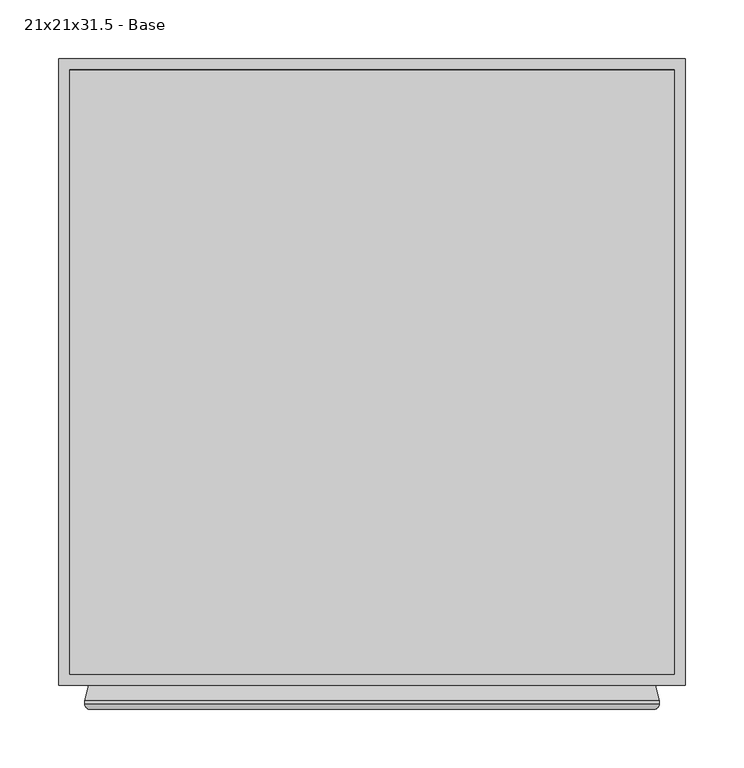
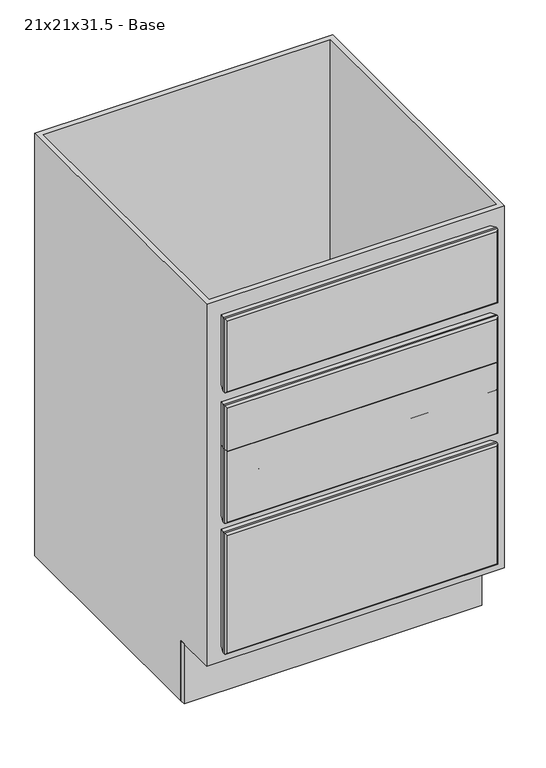
"""IFC4 building model written with IfcOpenShell, lengths in millimetres: furniture geometry, Cabinet-Base-Merillat-Four_Drawer-Marlin : 21x21x31.5 - Base."""

from ifc_helpers import new_model, si_unit, frame, origin, origin_with_axes, place, context, project, spatial, polyline, ellipse_curve, outline, extrude, faceted_brep, source, transform, mapped, element, save
from ifc_brep_helpers import plane_surface, cylinder_surface, advanced_brep


def furniture_21x21x31_5_base_fe1b8182(model_context):
    return source(origin(), model_context, "Body", "SolidModel", [
        advanced_brep(
        [(-222.6408026, -629.92, 365.2035075), (-222.6408026, -629.92, 142.7964925), (260.1162124, -629.92, 142.7964925), (260.1162124, -629.92, 365.2035075), (-222.2320951, -609.6, 143.2052), (-222.2320951, -609.6, 364.7948), (259.7075049, -609.6, 364.7948), (259.7075049, -609.6, 143.2052), (-225.7372951, -625.4496, 368.3), (-225.7372951, -622.681, 368.3), (-225.7372951, -622.681, 139.7), (-225.7372951, -625.4496, 139.7), (263.2127049, -622.681, 139.7), (263.2127049, -625.4496, 139.7), (263.2127049, -622.681, 368.3), (263.2127049, -625.4496, 368.3)],
        [
            (0, 1),
            (1, 2),
            (2, 3),
            (3, 0),
            (4, 5),
            (5, 6),
            (6, 7),
            (7, 4),
            (8, 9),
            (9, 10),
            (10, 11),
            (11, 8),
            (10, 12),
            (12, 13),
            (13, 11),
            (12, 14),
            (14, 15),
            (15, 13),
            (8, 15),
            (14, 9),
            (11, 1, ellipse_curve(frame((-220.9620951, -625.4496, 144.4752), z_axis=(-0.7071067811865475, 0.0, 0.7071067811865475), x_axis=(-0.7071067811865474, 0.0, -0.7071067811865476)), 6.7531526, 4.7752)),
            (0, 8, ellipse_curve(frame((-220.9620951, -625.4496, 363.5248), z_axis=(-0.7071067811865475, 0.0, -0.7071067811865475), x_axis=(0.7071067811865474, 0.0, -0.7071067811865476)), 6.7531526, 4.7752)),
            (4, 10),
            (9, 5),
            (13, 2, ellipse_curve(frame((258.4375049, -625.4496, 144.4752), z_axis=(-0.7071067811865475, 0.0, -0.7071067811865475), x_axis=(0.7071067811865476, 0.0, -0.7071067811865474)), 6.7531526, 4.7752)),
            (7, 12),
            (15, 3, ellipse_curve(frame((258.4375049, -625.4496, 363.5248), z_axis=(0.7071067811865475, 0.0, -0.7071067811865475), x_axis=(0.7071067811865474, 0.0, 0.7071067811865476)), 6.7531526, 4.7752)),
            (6, 14),
        ],
        [
            plane_surface(frame((-225.7372951, -629.92, 368.3), z_axis=(0.0, -1.0, 0.0), x_axis=(0.0, 0.0, -1.0))),
            plane_surface(frame((-225.7372951, -609.6, 368.3), z_axis=(0.0, 1.0, 0.0), x_axis=(0.0, 0.0, 1.0))),
            plane_surface(frame((-225.7372951, -629.92, 368.3), z_axis=(-1.0, 0.0, 0.0), x_axis=(0.0, 1.0, 0.0))),
            plane_surface(frame((-225.7372951, -629.92, 139.7), z_axis=(0.0, 0.0, -1.0), x_axis=(0.0, 1.0, 0.0))),
            plane_surface(frame((263.2127049, -629.92, 139.7), z_axis=(1.0, 0.0, 0.0), x_axis=(0.0, 1.0, 0.0))),
            plane_surface(frame((263.2127049, -629.92, 368.3), z_axis=(0.0, 0.0, 1.0), x_axis=(0.0, 1.0, 0.0))),
            cylinder_surface(frame((-220.9620951, -625.4496, 368.3), z_axis=(0.0, 0.0, -1.0), x_axis=(0.0, 1.0, 0.0)), 4.7752),
            plane_surface(frame((-225.7372951, -622.681, 368.3), z_axis=(-0.9659229350723619, 0.25882983502910506, 0.0), x_axis=(0.0, 0.0, -1.0))),
            cylinder_surface(frame((-225.7372951, -625.4496, 144.4752), z_axis=(1.0, 0.0, 0.0), x_axis=(0.0, 1.0, 0.0)), 4.7752),
            plane_surface(frame((-225.7372951, -622.681, 139.7), z_axis=(0.0, 0.25882983502910506, -0.9659229350723619), x_axis=(1.0, 0.0, 0.0))),
            cylinder_surface(frame((258.4375049, -625.4496, 139.7), z_axis=(0.0, 0.0, 1.0), x_axis=(0.0, 1.0, 0.0)), 4.7752),
            plane_surface(frame((263.2127049, -622.681, 139.7), z_axis=(0.9659229350723619, 0.25882983502910506, 0.0), x_axis=(0.0, 0.0, 1.0))),
            cylinder_surface(frame((263.2127049, -625.4496, 363.5248), z_axis=(-1.0, 0.0, 0.0), x_axis=(0.0, 1.0, 0.0)), 4.7752),
            plane_surface(frame((263.2127049, -622.681, 368.3), z_axis=(0.0, 0.25882983502910506, 0.9659229350723619), x_axis=(-1.0, 0.0, 0.0))),
        ],
        [
            (0, [[1, 2, 3, 4]]),
            (1, [[5, 6, 7, 8]]),
            (2, [[9, 10, 11, 12]]),
            (3, [[-11, 13, 14, 15]]),
            (4, [[-14, 16, 17, 18]]),
            (5, [[-9, 19, -17, 20]]),
            (6, [[21, -1, 22, -12]]),
            (7, [[23, -10, 24, -5]]),
            (8, [[-21, -15, 25, -2]]),
            (9, [[-23, -8, 26, -13]]),
            (10, [[-25, -18, 27, -3]]),
            (11, [[-26, -7, 28, -16]]),
            (12, [[-22, -4, -27, -19]]),
            (13, [[-24, -20, -28, -6]]),
        ],
    ),
        advanced_brep(
        [(-222.6408026, -629.92, 523.9535075), (-222.6408026, -629.92, 390.4464925), (260.1162124, -629.92, 390.4464925), (260.1162124, -629.92, 523.9535075), (-222.2320951, -609.6, 390.8552), (-222.2320951, -609.6, 523.5448), (259.7075049, -609.6, 523.5448), (259.7075049, -609.6, 390.8552), (-225.7372951, -625.4496, 527.05), (-225.7372951, -622.681, 527.05), (-225.7372951, -622.681, 387.35), (-225.7372951, -625.4496, 387.35), (263.2127049, -622.681, 387.35), (263.2127049, -625.4496, 387.35), (263.2127049, -622.681, 527.05), (263.2127049, -625.4496, 527.05)],
        [
            (0, 1),
            (1, 2),
            (2, 3),
            (3, 0),
            (4, 5),
            (5, 6),
            (6, 7),
            (7, 4),
            (8, 9),
            (9, 10),
            (10, 11),
            (11, 8),
            (10, 12),
            (12, 13),
            (13, 11),
            (12, 14),
            (14, 15),
            (15, 13),
            (8, 15),
            (14, 9),
            (11, 1, ellipse_curve(frame((-220.9620951, -625.4496, 392.1252), z_axis=(-0.7071067811865475, 0.0, 0.7071067811865475), x_axis=(-0.7071067811865474, 0.0, -0.7071067811865476)), 6.7531526, 4.7752)),
            (0, 8, ellipse_curve(frame((-220.9620951, -625.4496, 522.2748), z_axis=(-0.7071067811865475, 0.0, -0.7071067811865475), x_axis=(0.7071067811865474, 0.0, -0.7071067811865476)), 6.7531526, 4.7752)),
            (4, 10),
            (9, 5),
            (13, 2, ellipse_curve(frame((258.4375049, -625.4496, 392.1252), z_axis=(-0.7071067811865475, 0.0, -0.7071067811865475), x_axis=(0.7071067811865476, 0.0, -0.7071067811865474)), 6.7531526, 4.7752)),
            (7, 12),
            (15, 3, ellipse_curve(frame((258.4375049, -625.4496, 522.2748), z_axis=(0.7071067811865475, 0.0, -0.7071067811865475), x_axis=(0.7071067811865474, 0.0, 0.7071067811865476)), 6.7531526, 4.7752)),
            (6, 14),
        ],
        [
            plane_surface(frame((-225.7372951, -629.92, 527.05), z_axis=(0.0, -1.0, 0.0), x_axis=(0.0, 0.0, -1.0))),
            plane_surface(frame((-225.7372951, -609.6, 527.05), z_axis=(0.0, 1.0, 0.0), x_axis=(0.0, 0.0, 1.0))),
            plane_surface(frame((-225.7372951, -629.92, 527.05), z_axis=(-1.0, 0.0, 0.0), x_axis=(0.0, 1.0, 0.0))),
            plane_surface(frame((-225.7372951, -629.92, 387.35), z_axis=(0.0, 0.0, -1.0), x_axis=(0.0, 1.0, 0.0))),
            plane_surface(frame((263.2127049, -629.92, 387.35), z_axis=(1.0, 0.0, 0.0), x_axis=(0.0, 1.0, 0.0))),
            plane_surface(frame((263.2127049, -629.92, 527.05), z_axis=(0.0, 0.0, 1.0), x_axis=(0.0, 1.0, 0.0))),
            cylinder_surface(frame((-220.9620951, -625.4496, 527.05), z_axis=(0.0, 0.0, -1.0), x_axis=(0.0, 1.0, 0.0)), 4.7752),
            plane_surface(frame((-225.7372951, -622.681, 527.05), z_axis=(-0.9659229350723619, 0.25882983502910506, 0.0), x_axis=(0.0, 0.0, -1.0))),
            cylinder_surface(frame((-225.7372951, -625.4496, 392.1252), z_axis=(1.0, 0.0, 0.0), x_axis=(0.0, 1.0, 0.0)), 4.7752),
            plane_surface(frame((-225.7372951, -622.681, 387.35), z_axis=(0.0, 0.25882983502910506, -0.9659229350723619), x_axis=(1.0, 0.0, 0.0))),
            cylinder_surface(frame((258.4375049, -625.4496, 387.35), z_axis=(0.0, 0.0, 1.0), x_axis=(0.0, 1.0, 0.0)), 4.7752),
            plane_surface(frame((263.2127049, -622.681, 387.35), z_axis=(0.9659229350723619, 0.25882983502910506, 0.0), x_axis=(0.0, 0.0, 1.0))),
            cylinder_surface(frame((263.2127049, -625.4496, 522.2748), z_axis=(-1.0, 0.0, 0.0), x_axis=(0.0, 1.0, 0.0)), 4.7752),
            plane_surface(frame((263.2127049, -622.681, 527.05), z_axis=(0.0, 0.25882983502910506, 0.9659229350723619), x_axis=(-1.0, 0.0, 0.0))),
        ],
        [
            (0, [[1, 2, 3, 4]]),
            (1, [[5, 6, 7, 8]]),
            (2, [[9, 10, 11, 12]]),
            (3, [[-11, 13, 14, 15]]),
            (4, [[-14, 16, 17, 18]]),
            (5, [[-9, 19, -17, 20]]),
            (6, [[21, -1, 22, -12]]),
            (7, [[23, -10, 24, -5]]),
            (8, [[-21, -15, 25, -2]]),
            (9, [[-23, -8, 26, -13]]),
            (10, [[-25, -18, 27, -3]]),
            (11, [[-26, -7, 28, -16]]),
            (12, [[-22, -4, -27, -19]]),
            (13, [[-24, -20, -28, -6]]),
        ],
    ),
        advanced_brep(
        [(-222.6408026, -629.92, 606.5035075), (-222.6408026, -629.92, 472.9964925), (260.1162124, -629.92, 472.9964925), (260.1162124, -629.92, 606.5035075), (-222.2320951, -609.6, 473.4052), (-222.2320951, -609.6, 606.0948), (259.7075049, -609.6, 606.0948), (259.7075049, -609.6, 473.4052), (-225.7372951, -625.4496, 609.6), (-225.7372951, -622.681, 609.6), (-225.7372951, -622.681, 469.9), (-225.7372951, -625.4496, 469.9), (263.2127049, -622.681, 469.9), (263.2127049, -625.4496, 469.9), (263.2127049, -622.681, 609.6), (263.2127049, -625.4496, 609.6)],
        [
            (0, 1),
            (1, 2),
            (2, 3),
            (3, 0),
            (4, 5),
            (5, 6),
            (6, 7),
            (7, 4),
            (8, 9),
            (9, 10),
            (10, 11),
            (11, 8),
            (10, 12),
            (12, 13),
            (13, 11),
            (12, 14),
            (14, 15),
            (15, 13),
            (8, 15),
            (14, 9),
            (11, 1, ellipse_curve(frame((-220.9620951, -625.4496, 474.6752), z_axis=(-0.7071067811865475, 0.0, 0.7071067811865475), x_axis=(-0.7071067811865474, 0.0, -0.7071067811865476)), 6.7531526, 4.7752)),
            (0, 8, ellipse_curve(frame((-220.9620951, -625.4496, 604.8248), z_axis=(-0.7071067811865475, 0.0, -0.7071067811865475), x_axis=(0.7071067811865474, 0.0, -0.7071067811865476)), 6.7531526, 4.7752)),
            (4, 10),
            (9, 5),
            (13, 2, ellipse_curve(frame((258.4375049, -625.4496, 474.6752), z_axis=(-0.7071067811865475, 0.0, -0.7071067811865475), x_axis=(0.7071067811865476, 0.0, -0.7071067811865474)), 6.7531526, 4.7752)),
            (7, 12),
            (15, 3, ellipse_curve(frame((258.4375049, -625.4496, 604.8248), z_axis=(0.7071067811865475, 0.0, -0.7071067811865475), x_axis=(0.7071067811865474, 0.0, 0.7071067811865476)), 6.7531526, 4.7752)),
            (6, 14),
        ],
        [
            plane_surface(frame((-225.7372951, -629.92, 609.6), z_axis=(0.0, -1.0, 0.0), x_axis=(0.0, 0.0, -1.0))),
            plane_surface(frame((-225.7372951, -609.6, 609.6), z_axis=(0.0, 1.0, 0.0), x_axis=(0.0, 0.0, 1.0))),
            plane_surface(frame((-225.7372951, -629.92, 609.6), z_axis=(-1.0, 0.0, 0.0), x_axis=(0.0, 1.0, 0.0))),
            plane_surface(frame((-225.7372951, -629.92, 469.9), z_axis=(0.0, 0.0, -1.0), x_axis=(0.0, 1.0, 0.0))),
            plane_surface(frame((263.2127049, -629.92, 469.9), z_axis=(1.0, 0.0, 0.0), x_axis=(0.0, 1.0, 0.0))),
            plane_surface(frame((263.2127049, -629.92, 609.6), z_axis=(0.0, 0.0, 1.0), x_axis=(0.0, 1.0, 0.0))),
            cylinder_surface(frame((-220.9620951, -625.4496, 609.6), z_axis=(0.0, 0.0, -1.0), x_axis=(0.0, 1.0, 0.0)), 4.7752),
            plane_surface(frame((-225.7372951, -622.681, 609.6), z_axis=(-0.9659229350723619, 0.25882983502910506, 0.0), x_axis=(0.0, 0.0, -1.0))),
            cylinder_surface(frame((-225.7372951, -625.4496, 474.6752), z_axis=(1.0, 0.0, 0.0), x_axis=(0.0, 1.0, 0.0)), 4.7752),
            plane_surface(frame((-225.7372951, -622.681, 469.9), z_axis=(0.0, 0.25882983502910506, -0.9659229350723619), x_axis=(1.0, 0.0, 0.0))),
            cylinder_surface(frame((258.4375049, -625.4496, 469.9), z_axis=(0.0, 0.0, 1.0), x_axis=(0.0, 1.0, 0.0)), 4.7752),
            plane_surface(frame((263.2127049, -622.681, 469.9), z_axis=(0.9659229350723619, 0.25882983502910506, 0.0), x_axis=(0.0, 0.0, 1.0))),
            cylinder_surface(frame((263.2127049, -625.4496, 604.8248), z_axis=(-1.0, 0.0, 0.0), x_axis=(0.0, 1.0, 0.0)), 4.7752),
            plane_surface(frame((263.2127049, -622.681, 609.6), z_axis=(0.0, 0.25882983502910506, 0.9659229350723619), x_axis=(-1.0, 0.0, 0.0))),
        ],
        [
            (0, [[1, 2, 3, 4]]),
            (1, [[5, 6, 7, 8]]),
            (2, [[9, 10, 11, 12]]),
            (3, [[-11, 13, 14, 15]]),
            (4, [[-14, 16, 17, 18]]),
            (5, [[-9, 19, -17, 20]]),
            (6, [[21, -1, 22, -12]]),
            (7, [[23, -10, 24, -5]]),
            (8, [[-21, -15, 25, -2]]),
            (9, [[-23, -8, 26, -13]]),
            (10, [[-25, -18, 27, -3]]),
            (11, [[-26, -7, 28, -16]]),
            (12, [[-22, -4, -27, -19]]),
            (13, [[-24, -20, -28, -6]]),
        ],
    ),
        advanced_brep(
        [(-222.6408026, -629.92, 771.6035075), (-222.6408026, -629.92, 638.0964925), (260.1162124, -629.92, 638.0964925), (260.1162124, -629.92, 771.6035075), (-222.2320951, -609.6, 638.5052), (-222.2320951, -609.6, 771.1948), (259.7075049, -609.6, 771.1948), (259.7075049, -609.6, 638.5052), (-225.7372951, -625.4496, 774.7), (-225.7372951, -622.681, 774.7), (-225.7372951, -622.681, 635.0), (-225.7372951, -625.4496, 635.0), (263.2127049, -622.681, 635.0), (263.2127049, -625.4496, 635.0), (263.2127049, -622.681, 774.7), (263.2127049, -625.4496, 774.7)],
        [
            (0, 1),
            (1, 2),
            (2, 3),
            (3, 0),
            (4, 5),
            (5, 6),
            (6, 7),
            (7, 4),
            (8, 9),
            (9, 10),
            (10, 11),
            (11, 8),
            (10, 12),
            (12, 13),
            (13, 11),
            (12, 14),
            (14, 15),
            (15, 13),
            (8, 15),
            (14, 9),
            (11, 1, ellipse_curve(frame((-220.9620951, -625.4496, 639.7752), z_axis=(-0.7071067811865475, 0.0, 0.7071067811865475), x_axis=(-0.7071067811865474, 0.0, -0.7071067811865476)), 6.7531526, 4.7752)),
            (0, 8, ellipse_curve(frame((-220.9620951, -625.4496, 769.9248), z_axis=(-0.7071067811865475, 0.0, -0.7071067811865475), x_axis=(0.7071067811865474, 0.0, -0.7071067811865476)), 6.7531526, 4.7752)),
            (4, 10),
            (9, 5),
            (13, 2, ellipse_curve(frame((258.4375049, -625.4496, 639.7752), z_axis=(-0.7071067811865475, 0.0, -0.7071067811865475), x_axis=(0.7071067811865476, 0.0, -0.7071067811865474)), 6.7531526, 4.7752)),
            (7, 12),
            (15, 3, ellipse_curve(frame((258.4375049, -625.4496, 769.9248), z_axis=(0.7071067811865475, 0.0, -0.7071067811865475), x_axis=(0.7071067811865474, 0.0, 0.7071067811865476)), 6.7531526, 4.7752)),
            (6, 14),
        ],
        [
            plane_surface(frame((-225.7372951, -629.92, 774.7), z_axis=(0.0, -1.0, 0.0), x_axis=(0.0, 0.0, -1.0))),
            plane_surface(frame((-225.7372951, -609.6, 774.7), z_axis=(0.0, 1.0, 0.0), x_axis=(0.0, 0.0, 1.0))),
            plane_surface(frame((-225.7372951, -629.92, 774.7), z_axis=(-1.0, 0.0, 0.0), x_axis=(0.0, 1.0, 0.0))),
            plane_surface(frame((-225.7372951, -629.92, 635.0), z_axis=(0.0, 0.0, -1.0), x_axis=(0.0, 1.0, 0.0))),
            plane_surface(frame((263.2127049, -629.92, 635.0), z_axis=(1.0, 0.0, 0.0), x_axis=(0.0, 1.0, 0.0))),
            plane_surface(frame((263.2127049, -629.92, 774.7), z_axis=(0.0, 0.0, 1.0), x_axis=(0.0, 1.0, 0.0))),
            cylinder_surface(frame((-220.9620951, -625.4496, 774.7), z_axis=(0.0, 0.0, -1.0), x_axis=(0.0, 1.0, 0.0)), 4.7752),
            plane_surface(frame((-225.7372951, -622.681, 774.7), z_axis=(-0.9659229350723619, 0.25882983502910506, 0.0), x_axis=(0.0, 0.0, -1.0))),
            cylinder_surface(frame((-225.7372951, -625.4496, 639.7752), z_axis=(1.0, 0.0, 0.0), x_axis=(0.0, 1.0, 0.0)), 4.7752),
            plane_surface(frame((-225.7372951, -622.681, 635.0), z_axis=(0.0, 0.25882983502910506, -0.9659229350723619), x_axis=(1.0, 0.0, 0.0))),
            cylinder_surface(frame((258.4375049, -625.4496, 635.0), z_axis=(0.0, 0.0, 1.0), x_axis=(0.0, 1.0, 0.0)), 4.7752),
            plane_surface(frame((263.2127049, -622.681, 635.0), z_axis=(0.9659229350723619, 0.25882983502910506, 0.0), x_axis=(0.0, 0.0, 1.0))),
            cylinder_surface(frame((263.2127049, -625.4496, 769.9248), z_axis=(-1.0, 0.0, 0.0), x_axis=(0.0, 1.0, 0.0)), 4.7752),
            plane_surface(frame((263.2127049, -622.681, 774.7), z_axis=(0.0, 0.25882983502910506, 0.9659229350723619), x_axis=(-1.0, 0.0, 0.0))),
        ],
        [
            (0, [[1, 2, 3, 4]]),
            (1, [[5, 6, 7, 8]]),
            (2, [[9, 10, 11, 12]]),
            (3, [[-11, 13, 14, 15]]),
            (4, [[-14, 16, 17, 18]]),
            (5, [[-9, 19, -17, 20]]),
            (6, [[21, -1, 22, -12]]),
            (7, [[23, -10, 24, -5]]),
            (8, [[-21, -15, 25, -2]]),
            (9, [[-23, -8, 26, -13]]),
            (10, [[-25, -18, 27, -3]]),
            (11, [[-26, -7, 28, -16]]),
            (12, [[-22, -4, -27, -19]]),
            (13, [[-24, -20, -28, -6]]),
        ],
    ),
        extrude(outline(polyline([(285.4377049, -529.43125), (285.4377049, -538.95625), (-247.9622951, -538.95625), (-247.9622951, -529.43125), (285.4377049, -529.43125)])), origin_with_axes(), (0.0, 0.0, 1.0), 114.3),
        faceted_brep([(285.4377049, -76.2, 0.0), (285.4377049, -529.43125, 0.0), (275.9127049, -529.43125, 0.0), (275.9127049, -85.725, 0.0), (-238.4372951, -85.725, 0.0), (-238.4372951, -529.43125, 0.0), (-247.9622951, -529.43125, 0.0), (-247.9622951, -76.2, 0.0), (-247.9622951, -76.2, 800.1), (285.4377049, -76.2, 800.1), (-247.9622951, -529.43125, 114.3), (-247.9622951, -609.6, 114.3), (-247.9622951, -609.6, 800.1), (285.4377049, -609.6, 800.1), (285.4377049, -609.6, 114.3), (285.4377049, -529.43125, 114.3), (275.9127049, -529.43125, 114.3), (275.9127049, -85.725, 114.3), (275.9127049, -600.075, 800.1), (275.9127049, -85.725, 800.1), (275.9127049, -85.725, 119.0625), (275.9127049, -600.075, 119.0625), (-238.4372951, -85.725, 114.3), (-238.4372951, -529.43125, 114.3), (-238.4372951, -85.725, 800.1), (-238.4372951, -600.075, 800.1), (-238.4372951, -600.075, 119.0625), (-238.4372951, -85.725, 119.0625)], [[[0, 1, 2, 3, 4, 5, 6, 7]], [[0, 7, 8, 9]], [[7, 6, 10, 11, 12, 8]], [[1, 0, 9, 13, 14, 15]], [[3, 2, 16, 17]], [[18, 19, 20, 21]], [[5, 4, 22, 23]], [[24, 25, 26, 27]], [[4, 3, 17, 22]], [[19, 24, 27, 20]], [[9, 8, 12, 13], [19, 18, 25, 24]], [[14, 11, 10, 23, 22, 17, 16, 15]], [[13, 12, 11, 14]], [[25, 18, 21, 26]], [[6, 5, 23, 10]], [[2, 1, 15, 16]], [[21, 20, 27, 26]]]),
    ])


if __name__ == "__main__":
    model = new_model("IFC4")
    model_context = context("Model", 3, world=origin())
    ifc_project = project(units=[si_unit("LENGTHUNIT", "METRE", prefix="MILLI")], contexts=[model_context])
    site = spatial("IfcSite", under=ifc_project)
    building = spatial("IfcBuilding", under=site)
    placement = place(None, origin())
    furniture_21x21x31_5_base_shape = furniture_21x21x31_5_base_fe1b8182(model_context)
    element("IfcFurniture", 1, ObjectType="Cabinet-Base-Merillat-Four_Drawer-Marlin : 21x21x31.5 - Base", at=placement, inside=building, context=model_context, shape_type="MappedRepresentation", body=[
        mapped(furniture_21x21x31_5_base_shape, transform((0.0, 0.0, 0.0), x_axis=(1.0, 0.0, 0.0), y_axis=(0.0, 1.0, 0.0), z_axis=(0.0, 0.0, 1.0))),
    ])
    save(model, "model.ifc")

# Revit data of these elements
# Type "Cabinet-Base-Merillat-Four_Drawer-Marlin : 21x21x31.5 - Base"
#   URL = "http://www.merillat.com"
#   Toe Kick Note = "Toe Kick Covering is not included. To be purchased Separately."
#   Product Line = "Express"
#   Product Page URL = "http://www.merillat.com//our-products/rooms/kitchen/"
#   Product Group = "Base Cabinet"
#   Product Documentation Link = "http://merillatbusiness.com/customer-resources/product-line-resources/merillat-classic/"
#   Model = "BD21-4D"
#   Manufacturer = "Merillat"
#   Finish = "Wood"
#   Description = "Base Four Drawer Cabinet"
#   Construction Type = "Base Four Drawer"
#   Cabinet Construction Note = "3/4 extension sliders on all three drawers when SST or PST construction is chosen"
#   Assembly Code = "C1030410"
#   Top and Bottom Spacing = 0' - 1"
#   Toe Kick Height = 0' - 4 1/2"
#   Toe Kick Depth = 0' - 2 25/32"
#   Cabinet Shell = 0' - 0 3/8"
#   Middle Drawer Spacing = 0' - 0 3/4"
#   Depth = 1' - 9"
#   Height = 2' - 7 1/2"
#   Width = 1' - 9"
#   Deep Cabinet Drawer Height = 0' - 9"
#   Cabinet Drawer Width = 1' - 7 1/4"
#   Cabinet Drawer Height = 0' - 5 1/2"
#   COBie.Type = no
#   Partial Overlay = yes
#   Full Overlay = no
#   Toe Kick Material = Wood - Merillat - Raw Particle Board
#   Door Drawer Material = Wood - Merillat - Pecan(1)
#   Cabinet Drawer Style = element 826866
#   Cabinet Material = Wood - Merillat - Pecan(1)
# Element 1 (IfcFurniture, "Cabinet-Base-Merillat-Four_Drawer-Marlin : 21x21x31.5 - Base")
#   Materials on its faces: "Wood - Merillat - Pecan(1)", "Wood - Merillat - Raw Particle Board"
# Materials
#   "Wood - Merillat - Raw Particle Board": class "Plastic", colour RGB 80 80 80, transparency 0, Description = "Plastic Laminate - Navy", Cost = 0
#   "Wood - Merillat - Pecan(1)": class "Wood", colour RGB 108 67 43, transparency 0, Cost = 0
